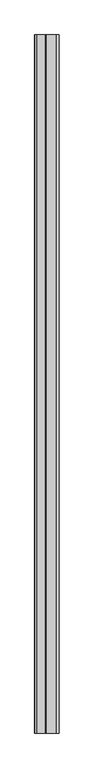
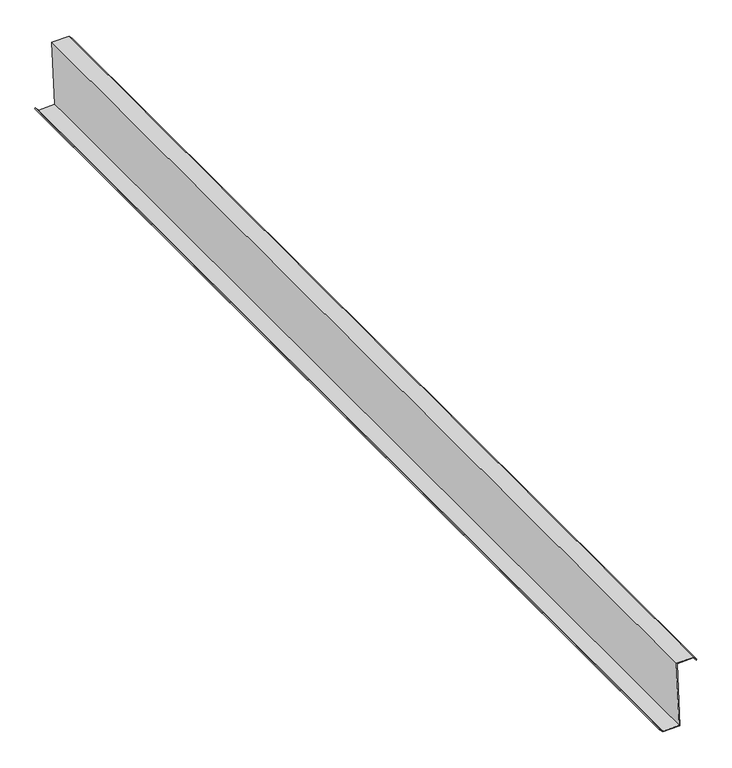
"""IFC4 building model written with IfcOpenShell, lengths in millimetres: proxy geometry, Generic Models 7:Generic Models 1:337419:Generic Models 1:337419 : Generic Models 7:Generic Models 1:337419:3 : Generic Models 7:Generic Models 1:337419:Generic Models 1:337419 : Generic Models 7:Generic Models 1:337419:301336."""

from ifc_helpers import new_model, si_unit, frame, origin, place, context, project, spatial, polyline, outline, extrude, source, transform, mapped, element, save


def generic_models_beb9be0c(model_context):
    return source(origin(), model_context, "Body", "SweptSolid", [
        extrude(outline(polyline([(4446.9250826, 579005.7215811), (4697.9291666, 578995.2630776), (4700.460948, 579056.0258315), (4687.1675522, 579068.158391), (4689.2198702, 579070.0465236), (4703.2905953, 579057.2045146), (4700.5892283, 578992.3717061), (4449.5851443, 579002.8302096), (4447.0533629, 578942.0674557), (4460.1672337, 578930.0987444), (4458.1149156, 578928.2106118), (4444.2237156, 578940.8887726), (4446.9250826, 579005.7215811)])), frame((0.0, -578746.6913841, 0.0), z_axis=(0.0, 1.0, 0.0), x_axis=(0.0, 0.0, 1.0)), (0.0, 0.0, 1.0), 4094.7624605),
    ])


if __name__ == "__main__":
    model = new_model("IFC4")
    model_context = context("Model", 3, world=origin())
    ifc_project = project(units=[si_unit("LENGTHUNIT", "METRE", prefix="MILLI")], contexts=[model_context])
    site = spatial("IfcSite", under=ifc_project)
    building = spatial("IfcBuilding", under=site)
    placement = place(None, origin())
    generic_models_shape = generic_models_beb9be0c(model_context)
    element("IfcBuildingElementProxy", 1, Name="Generic Models 7:Generic Models 1:337419:Generic Models 1:337419 : Generic Models 7:Generic Models 1:337419:3 : Generic Models 7:Generic Models 1:337419:Generic Models 1:337419 : Generic Models 7:Generic Models 1:337419:301336", ObjectType="Generic Models 7:Generic Models 1:337419:Generic Models 1:337419 : Generic Models 7:Generic Models 1:337419:3 : Generic Models 7:Generic Models 1:337419:Generic Models 1:337419 : Generic Models 7:Generic Models 1:337419:301336", at=placement, inside=building, context=model_context, shape_type="MappedRepresentation", body=[
        mapped(generic_models_shape, transform((0.0, 0.0, 0.0), x_axis=(1.0, 0.0, 0.0), y_axis=(0.0, 1.0, 0.0), z_axis=(0.0, 0.0, 1.0))),
    ])
    save(model, "model.ifc")

# Revit data of these elements
# Type "Generic Models 7:Generic Models 1:337419:Generic Models 1:337419 : Generic Models 7:Generic Models 1:337419:3 : Generic Models 7:Generic Models 1:337419:Generic Models 1:337419 : Generic Models 7:Generic Models 1:337419:301336"
#   NameOverride = "Generic Models 7:Generic Models 1:337419:Generic Models 1:337419 : Generic Models 7:Generic Models 1:337419:301336"
#   ObjectTypeOverride = "Generic Models 1:337419 : Generic Models 7:Generic Models 1:337419"
#   Reference = "Generic Models 1"
#   Tag = "301336"
# Element 1 (IfcBuildingElementProxy, "Generic Models 7:Generic Models 1:337419:Generic Models 1:337419 : Generic Models 7:Generic Models 1:337419:3 : Generic Models 7:Generic Models 1:337419:Generic Models 1:337419 : Generic Models 7:Generic Models 1:337419:301336")
#   Materials on its faces: "'ZEE' SECTION (8.0x3.5Z - SEE STRUCT. DWGS)"
# Materials
#   "'ZEE' SECTION (8.0x3.5Z - SEE STRUCT. DWGS)": class "Unassigned", colour RGB 210 209 208, transparency 0, Keynote = "M05121300.02", Cost = 0
